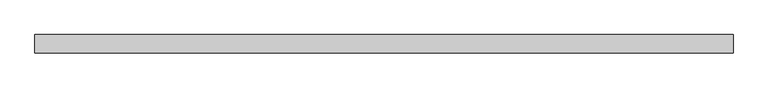
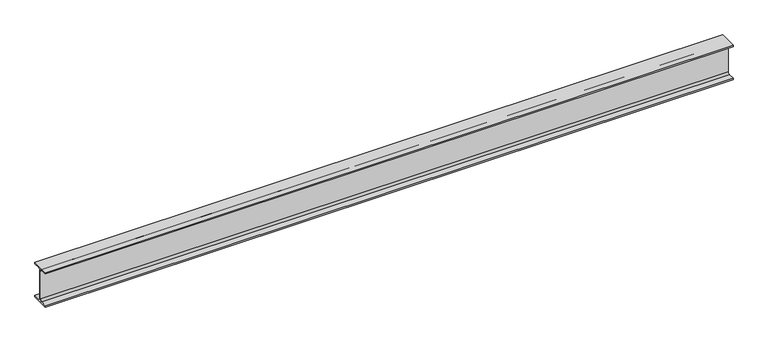
"""IFC4 building model written with IfcOpenShell, lengths in millimetres: beam geometry, 0912_Steel Framing_H-KSD3502 : H_SB_H-200x100x5.5x8."""

from ifc_helpers import new_model, si_unit, point, frame, frame_2d, origin, place, context, project, spatial, polyline, circle_curve, trimmed, segment, composite_curve, outline, extrude, source, transform, mapped, element, save


def beam_cef0ad3f(model_context):
    return source(origin(), model_context, "Body", "SweptSolid", [
        extrude(outline(composite_curve([segment(polyline([(50.0, -92.0), (50.0, -100.0), (-50.0, -100.0), (-50.0, -92.0), (-13.75, -92.0)]), True, "CONTINUOUS"), segment(trimmed(circle_curve(frame_2d((-13.75, -81.0)), 11.0), [point((-13.75, -92.0))], [point((-2.75, -81.0))], True, "CARTESIAN"), True, "CONTINUOUS"), segment(polyline([(-2.75, -81.0), (-2.75, 81.0)]), True, "CONTINUOUS"), segment(trimmed(circle_curve(frame_2d((-13.75, 81.0)), 11.0), [point((-2.75, 81.0))], [point((-13.75, 92.0))], True, "CARTESIAN"), True, "CONTINUOUS"), segment(polyline([(-13.75, 92.0), (-50.0, 92.0), (-50.0, 100.0), (50.0, 100.0), (50.0, 92.0), (13.75, 92.0)]), True, "CONTINUOUS"), segment(trimmed(circle_curve(frame_2d((13.75, 81.0)), 11.0), [point((13.75, 92.0))], [point((2.75, 81.0))], True, "CARTESIAN"), True, "CONTINUOUS"), segment(polyline([(2.75, 81.0), (2.75, -81.0)]), True, "CONTINUOUS"), segment(trimmed(circle_curve(frame_2d((13.75, -81.0)), 11.0), [point((2.75, -81.0))], [point((13.75, -92.0))], True, "CARTESIAN"), True, "CONTINUOUS"), segment(polyline([(13.75, -92.0), (50.0, -92.0)]), True, "CONTINUOUS")], self_intersect=False)), frame((-1887.3, 0.0, 0.0), z_axis=(1.0, 0.0, 0.0), x_axis=(0.0, 1.0, 0.0)), (0.0, 0.0, 1.0), 3774.6),
    ])


if __name__ == "__main__":
    model = new_model("IFC4")
    model_context = context("Model", 3, world=origin())
    ifc_project = project(units=[si_unit("LENGTHUNIT", "METRE", prefix="MILLI")], contexts=[model_context])
    site = spatial("IfcSite", under=ifc_project)
    building = spatial("IfcBuilding", under=site)
    placement = place(None, origin())
    beam_shape = beam_cef0ad3f(model_context)
    element("IfcBeam", 1, ObjectType="0912_Steel Framing_H-KSD3502 : H_SB_H-200x100x5.5x8", at=placement, inside=building, context=model_context, shape_type="MappedRepresentation", body=[
        mapped(beam_shape, transform((0.0, 0.0, 0.0), x_axis=(1.0, 0.0, 0.0), y_axis=(0.0, 1.0, 0.0), z_axis=(0.0, 0.0, 1.0))),
    ])
    save(model, "model.ifc")

# Revit data of these elements
# Type "0912_Steel Framing_H-KSD3502 : H_SB_H-200x100x5.5x8"
#   Width = 10.0 cm
#   Web Thickness = 0.55 cm
#   Web Fillet = 1.1 cm
#   Warping Constant = 12288.0 cm⁶
#   W = 0
#   Torsional Moment of Inertia = 4.4781 cm⁴
#   Section Area = 27.16 cm²
#   Plastic Modulus weak axis = 41.9 cm³
#   Plastic Modulus strong axis = 209.0 cm³
#   Perimeter = 0.77 m²/m
#   Nominal Weight = 21.30 kgf/m
#   Moment of Inertia weak axis = 134.00 cm⁴
#   Moment of Inertia strong axis = 1840.00 cm⁴
#   Height = 20.0 cm
#   Flange Thickness = 0.8 cm
#   Elastic Modulus weak axis = 26.8 cm³
#   Elastic Modulus strong axis = 184.0 cm³
#   Centroid Vertical = 10.0 cm
#   Centroid Horizontal = 5.0 cm
#   Ix = 18400000
#   Length [instance default] = 1524 mm
#   Zx = 209000
#   b = 100 mm
#   h = 200 mm
#   r = 11 mm
#   s = 5.5 mm
#   t = 8 mm
#   A = 0.002716 m²
#   Structural Material [instance default] = Steel, 45-345
#   Assembly Code = ""
# Element 1 (IfcBeam, "0912_Steel Framing_H-KSD3502 : H_SB_H-200x100x5.5x8")
#   Materials on its faces: "Steel, 45-345"
# Materials
#   "Steel, 45-345": class "Metal", colour RGB 189 187 185, transparency 0, Description = "Steel 345 MPa", Cost = 0
